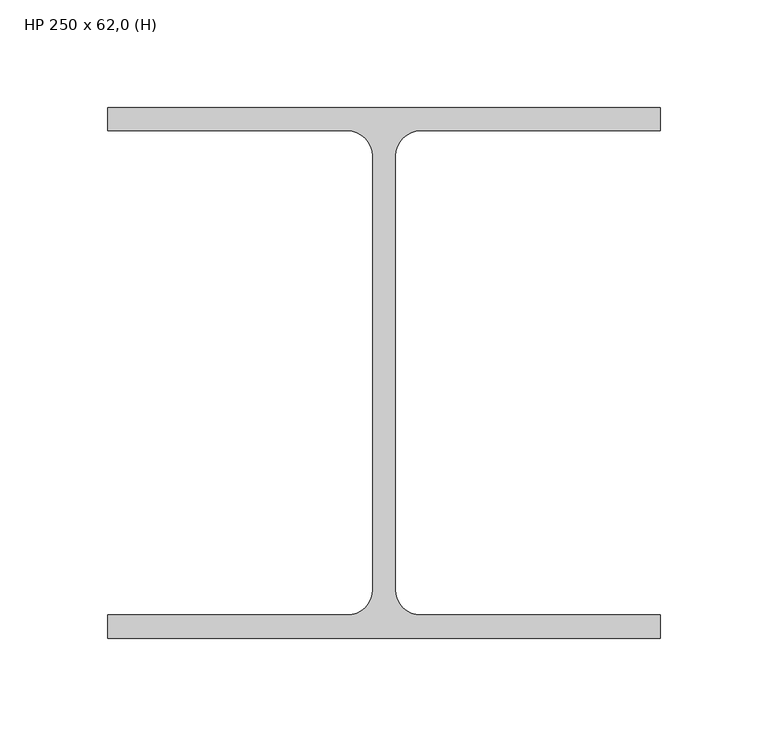
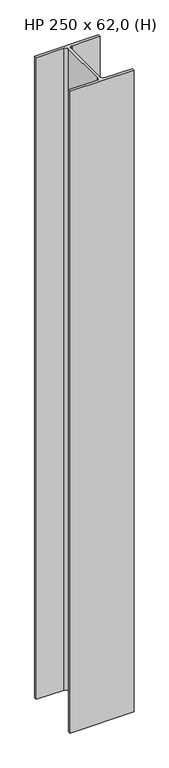
"""IFC4 building model written with IfcOpenShell, lengths in millimetres: column geometry, Pilar de Aço - H : HP 250 x 62,0 (H)."""

from ifc_helpers import new_model, si_unit, point, frame_2d, origin, origin_with_axes, place, context, project, spatial, polyline, circle_curve, trimmed, segment, composite_curve, outline, extrude, source, transform, mapped, element, save


def hp_250_x_62_0_h_a9bd0f42(model_context):
    return source(origin(), model_context, "Body", "SweptSolid", [
        extrude(outline(composite_curve([segment(polyline([(128.0, 123.0), (128.0, 112.3), (17.05, 112.3)]), True, "CONTINUOUS"), segment(trimmed(circle_curve(frame_2d((17.05, 100.5)), 11.8), [point((17.05, 112.3))], [point((5.25, 100.5))], True, "CARTESIAN"), True, "CONTINUOUS"), segment(polyline([(5.25, 100.5), (5.25, -100.5)]), True, "CONTINUOUS"), segment(trimmed(circle_curve(frame_2d((17.05, -100.5)), 11.8), [point((5.25, -100.5))], [point((17.05, -112.3))], True, "CARTESIAN"), True, "CONTINUOUS"), segment(polyline([(17.05, -112.3), (128.0, -112.3), (128.0, -123.0), (-128.0, -123.0), (-128.0, -112.3), (-17.05, -112.3)]), True, "CONTINUOUS"), segment(trimmed(circle_curve(frame_2d((-17.05, -100.5)), 11.8), [point((-17.05, -112.3))], [point((-5.25, -100.5))], True, "CARTESIAN"), True, "CONTINUOUS"), segment(polyline([(-5.25, -100.5), (-5.25, 100.5)]), True, "CONTINUOUS"), segment(trimmed(circle_curve(frame_2d((-17.05, 100.5)), 11.8), [point((-5.25, 100.5))], [point((-17.05, 112.3))], True, "CARTESIAN"), True, "CONTINUOUS"), segment(polyline([(-17.05, 112.3), (-128.0, 112.3), (-128.0, 123.0), (128.0, 123.0)]), True, "CONTINUOUS")], self_intersect=False)), origin_with_axes(), (0.0, 0.0, 1.0), 2720.0),
    ])


if __name__ == "__main__":
    model = new_model("IFC4")
    model_context = context("Model", 3, world=origin())
    ifc_project = project(units=[si_unit("LENGTHUNIT", "METRE", prefix="MILLI")], contexts=[model_context])
    site = spatial("IfcSite", under=ifc_project)
    building = spatial("IfcBuilding", under=site)
    placement = place(None, origin())
    hp_250_x_62_0_h_shape = hp_250_x_62_0_h_a9bd0f42(model_context)
    element("IfcColumn", 1, ObjectType="Pilar de Aço - H : HP 250 x 62,0 (H)", at=placement, inside=building, context=model_context, shape_type="MappedRepresentation", body=[
        mapped(hp_250_x_62_0_h_shape, transform((0.0, 0.0, 0.0), x_axis=(1.0, 0.0, 0.0), y_axis=(0.0, 1.0, 0.0), z_axis=(0.0, 0.0, 1.0))),
    ])
    save(model, "model.ifc")

# Revit data of these elements
# Type "Pilar de Aço - H : HP 250 x 62,0 (H)"
#   SINAPI = ""
#   Área da seção = 79.6 m²
#   tw = 1.05 cm
#   tf = 1.07 cm
#   h = 22.46 cm
#   d' = 20.10 cm
#   d = 24.60 cm
#   bf = 25.60 cm
#   R = 1.18 cm
#   Massa Linear kg/m = 62
#   Aço = Metal - Aço 345MPa
#   Assembly Code = ""
# Materials
#   "Metal - Aço 345MPa": class "Metal", colour RGB 189 187 185, transparency 0, Cost = 0
